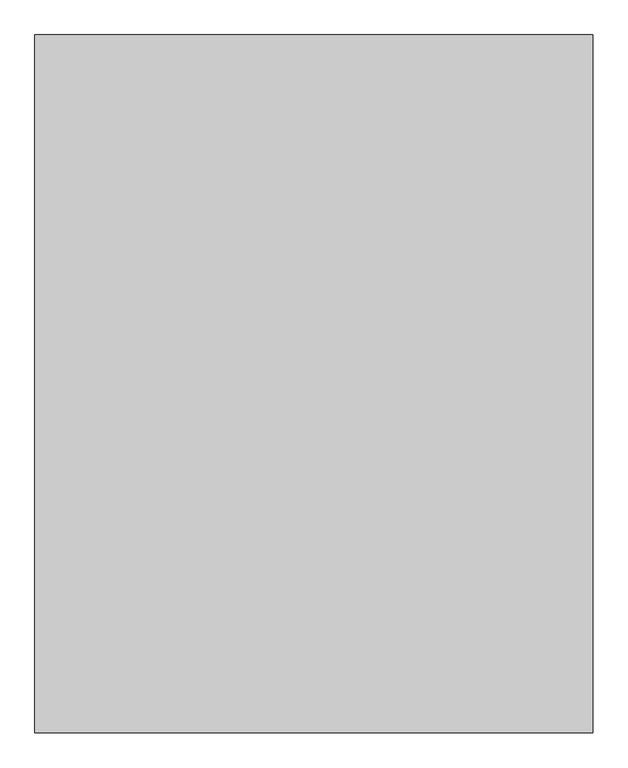
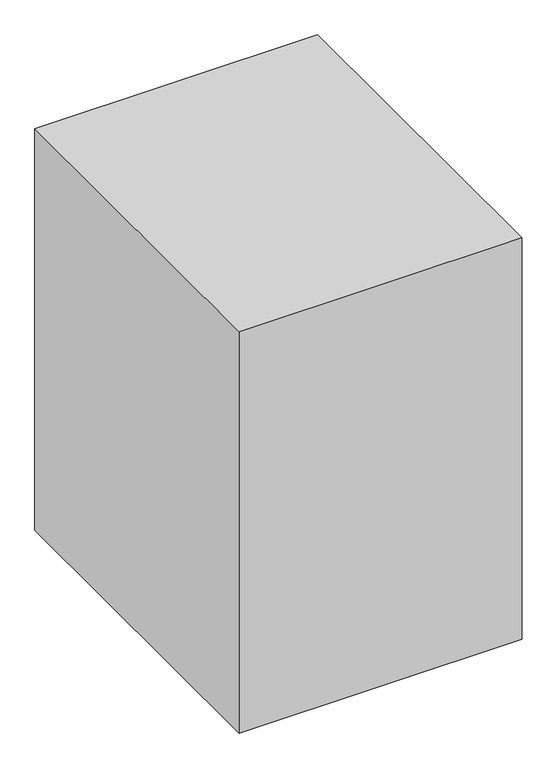
"""IFC4 building model written with IfcOpenShell, lengths in millimetres: proxy geometry, Space Planning Box_hec : Space Planning Box_hec."""

import ifcopenshell
import ifcopenshell.guid

model = None  # the IFC model being written
_history = None  # IfcOwnerHistory: only IFC2X3 demands one
_inside = {}  # id of a spatial element -> (the spatial element, [elements in it])
_under = {}  # id of a project, library or spatial element -> (it, [spatial elements below it])
_declared = {}  # id of a project -> (the project, [libraries it declares])
_typed = {}  # id of a type object -> (the type object, [elements of that type])
_made_of = {}  # id of a material, layer set ... -> (it, [elements and type objects made of it])


def new_model(schema):
    """Start an empty IFC model of exactly this schema.

    Asked for "IFC4X3", IfcOpenShell would pick the latest addendum, in which some entities
    have other attributes; the version numbers below select the first issue.
    IFC2X3 requires an IfcOwnerHistory on every rooted entity: one is made here for all.
    """
    global model, _history
    if schema == "IFC4X3":
        model = ifcopenshell.file(schema_version=(4, 3, 0, 0))
    else:
        model = ifcopenshell.file(schema=schema)
    _inside.clear()
    _under.clear()
    _declared.clear()
    _typed.clear()
    _made_of.clear()
    _history = None
    if model.schema == "IFC2X3":
        org = make("IfcOrganization", Name="unknown")
        user = make(
            "IfcPersonAndOrganization",
            ThePerson=make("IfcPerson", FamilyName="unknown"),
            TheOrganization=org,
        )
        app = make(
            "IfcApplication",
            ApplicationDeveloper=org,
            Version="unknown",
            ApplicationFullName="unknown",
            ApplicationIdentifier="unknown",
        )
        _history = make(
            "IfcOwnerHistory",
            OwningUser=user,
            OwningApplication=app,
            ChangeAction="ADDED",
            CreationDate=0,
        )
    return model


def make(cls, **values):
    """One entity of the class cls with the attributes given. An attribute that is None is left unset."""
    return model.create_entity(
        cls, **{name: value for name, value in values.items() if value is not None}
    )


def rooted(cls, **values):
    """An entity with a GlobalId (a new one), such as an element, a storey or a relation."""
    return make(cls, GlobalId=ifcopenshell.guid.new(), OwnerHistory=_history, **values)


def si_unit(unit_type, name, prefix=None):
    """IfcSIUnit, for example si_unit("LENGTHUNIT", "METRE", prefix="MILLI")."""
    return make("IfcSIUnit", UnitType=unit_type, Prefix=prefix, Name=name)


def assignment(units):
    """IfcUnitAssignment: the units of a project."""
    return None if units is None else make("IfcUnitAssignment", Units=units)


def point(xyz):
    """IfcCartesianPoint."""
    return None if xyz is None else make("IfcCartesianPoint", Coordinates=xyz)


def direction(xyz):
    """IfcDirection."""
    return None if xyz is None else make("IfcDirection", DirectionRatios=xyz)


def frame(location, z_axis=None, x_axis=None):
    """IfcAxis2Placement3D, a coordinate frame: its origin and axes. An axis left out is left unset."""
    return make(
        "IfcAxis2Placement3D",
        Location=point(location),
        Axis=direction(z_axis),
        RefDirection=direction(x_axis),
    )


def origin():
    """The frame at (0, 0, 0) with its axes left unset."""
    return frame((0.0, 0.0, 0.0))


def origin_with_axes():
    """The frame at (0, 0, 0) with the z axis (0, 0, 1) and the x axis (1, 0, 0) written out."""
    return frame((0.0, 0.0, 0.0), z_axis=(0.0, 0.0, 1.0), x_axis=(1.0, 0.0, 0.0))


def place(relative_to, where):
    """IfcLocalPlacement: puts the frame where relative to a parent placement (None: the world)."""
    return make(
        "IfcLocalPlacement", PlacementRelTo=relative_to, RelativePlacement=where
    )


def context(
    kind, dimensions, precision=None, world=None, true_north=None, identifier=None
):
    """IfcGeometricRepresentationContext, for example the 3D "Model" context."""
    return make(
        "IfcGeometricRepresentationContext",
        ContextIdentifier=identifier,
        ContextType=kind,
        CoordinateSpaceDimension=dimensions,
        Precision=precision,
        WorldCoordinateSystem=world,
        TrueNorth=true_north,
    )


def project(units=None, contexts=None):
    """IfcProject with its units and contexts."""
    return rooted(
        "IfcProject",
        Name="project",
        RepresentationContexts=contexts,
        UnitsInContext=assignment(units),
    )


def spatial(cls, under=None, at=None, **own):
    """A site, building, storey or space (cls), placed at a placement, below another one or the project."""
    s = rooted(cls, ObjectPlacement=at, **own)
    if under is not None:
        _under.setdefault(under.id(), (under, []))[1].append(s)
    return s


def polyline(points):
    """IfcPolyline through the points."""
    return make("IfcPolyline", Points=[point(p) for p in points])


def outline(outer, holes=None, kind="AREA"):
    """IfcArbitraryClosedProfileDef: a profile drawn as a closed curve; with holes, ...WithVoids."""
    if holes is None:
        return make("IfcArbitraryClosedProfileDef", ProfileType=kind, OuterCurve=outer)
    return make(
        "IfcArbitraryProfileDefWithVoids",
        ProfileType=kind,
        OuterCurve=outer,
        InnerCurves=holes,
    )


def extrude(swept, where, along, depth):
    """IfcExtrudedAreaSolid: the profile swept, set in the frame where, extruded along a direction by depth."""
    return make(
        "IfcExtrudedAreaSolid",
        SweptArea=swept,
        Position=where,
        ExtrudedDirection=direction(along),
        Depth=depth,
    )


def shape(context_of_items, identifier, shape_type, items):
    """IfcShapeRepresentation: the items that make up one representation, for example the "Body"."""
    return make(
        "IfcShapeRepresentation",
        ContextOfItems=context_of_items,
        RepresentationIdentifier=identifier,
        RepresentationType=shape_type,
        Items=items,
    )


def source(mapping_origin, context_of_items, identifier, shape_type, items):
    """IfcRepresentationMap: a shape defined once, which mapped items show again and again."""
    return make(
        "IfcRepresentationMap",
        MappingOrigin=mapping_origin,
        MappedRepresentation=shape(context_of_items, identifier, shape_type, items),
    )


def transform(
    local_origin,
    x_axis=None,
    y_axis=None,
    z_axis=None,
    scale=None,
    scale2=None,
    scale3=None,
    uniform=True,
):
    """IfcCartesianTransformationOperator3D, or its non-uniform kind. x_axis, y_axis, z_axis: its Axis1, 2, 3."""
    if uniform:
        return make(
            "IfcCartesianTransformationOperator3D",
            Axis1=direction(x_axis),
            Axis2=direction(y_axis),
            LocalOrigin=point(local_origin),
            Scale=scale,
            Axis3=direction(z_axis),
        )
    return make(
        "IfcCartesianTransformationOperator3DnonUniform",
        Axis1=direction(x_axis),
        Axis2=direction(y_axis),
        LocalOrigin=point(local_origin),
        Scale=scale,
        Axis3=direction(z_axis),
        Scale2=scale2,
        Scale3=scale3,
    )


def mapped(mapping_source, mapping_target):
    """IfcMappedItem: shows the shape of a source again, moved by a transform."""
    return make(
        "IfcMappedItem", MappingSource=mapping_source, MappingTarget=mapping_target
    )


def made_of(thing, what):
    """Note that an element or type object is made of a material, layer set ...; save() writes the relation."""
    if what is not None:
        _made_of.setdefault(what.id(), (what, []))[1].append(thing)
    return thing


def element(
    cls,
    number,
    at=None,
    inside=None,
    cuts=None,
    type_object=None,
    material=None,
    context=None,
    identifier="Body",
    shape_type=None,
    held_by="IfcProductDefinitionShape",
    body=None,
    shapes=None,
    **own,
):
    """One element of the class cls, such as IfcWall. Its Tag is "e" and its number.

    at: its placement. inside: the storey or other place that contains it. cuts: it is an
    opening in that element (IfcRelVoidsElement). A single representation is given by context,
    identifier, shape_type and body (its items); several are given by shapes. held_by: the class
    of the entity that holds the representations. save() writes the other relations.
    """
    e = rooted(cls, Tag="e%d" % number, ObjectPlacement=at, **own)
    if body is not None:
        shapes = [shape(context, identifier, shape_type, body)]
    if shapes is not None:
        e.Representation = make(held_by, Representations=shapes)
    if inside is not None:
        _inside.setdefault(inside.id(), (inside, []))[1].append(e)
    if cuts is not None:
        rooted(
            "IfcRelVoidsElement", RelatingBuildingElement=cuts, RelatedOpeningElement=e
        )
    if type_object is not None:
        _typed.setdefault(type_object.id(), (type_object, []))[1].append(e)
    return made_of(e, material)


def aggregate(whole, parts):
    """IfcRelAggregates: a whole, such as a stair, and the parts it consists of."""
    return rooted("IfcRelAggregates", RelatingObject=whole, RelatedObjects=parts)


def save(model, path):
    """Write the relations noted so far, then the file.

    IfcRelAggregates (storeys below a building ...), IfcRelContainedInSpatialStructure (elements
    in a storey), IfcRelDefinesByType, IfcRelAssociatesMaterial and IfcRelDeclares: one each for
    every whole, place, type object, material and project.
    """
    for whole, parts in _under.values():
        aggregate(whole, parts)
    for where, things in _inside.values():
        rooted(
            "IfcRelContainedInSpatialStructure",
            RelatedElements=things,
            RelatingStructure=where,
        )
    for kind, things in _typed.values():
        rooted("IfcRelDefinesByType", RelatedObjects=things, RelatingType=kind)
    for what, things in _made_of.values():
        rooted("IfcRelAssociatesMaterial", RelatedObjects=things, RelatingMaterial=what)
    for by, libraries in _declared.values():
        rooted("IfcRelDeclares", RelatingContext=by, RelatedDefinitions=libraries)
    model.write(path)


def generic_models_5b7b272c(model_context):
    return source(origin(), model_context, "Body", "SweptSolid", [
        extrude(outline(polyline([(2000.0, 2500.0), (2000.0, -2500.0), (-2000.0, -2500.0), (-2000.0, 2500.0), (2000.0, 2500.0)])), origin_with_axes(), (0.0, 0.0, 1.0), 6000.0),
    ])


if __name__ == "__main__":
    model = new_model("IFC4")
    model_context = context("Model", 3, world=origin())
    ifc_project = project(units=[si_unit("LENGTHUNIT", "METRE", prefix="MILLI")], contexts=[model_context])
    site = spatial("IfcSite", under=ifc_project)
    building = spatial("IfcBuilding", under=site)
    placement = place(None, origin())
    generic_models_shape = generic_models_5b7b272c(model_context)
    element("IfcBuildingElementProxy", 1, Name="Space Planning Box_hec : Space Planning Box_hec", ObjectType="Space Planning Box_hec : Space Planning Box_hec", at=placement, inside=building, context=model_context, shape_type="MappedRepresentation", body=[
        mapped(generic_models_shape, transform((0.0, 0.0, 0.0), x_axis=(1.0, 0.0, 0.0), y_axis=(0.0, 1.0, 0.0), z_axis=(0.0, 0.0, 1.0))),
    ])
    save(model, "model.ifc")

# Revit data of these elements
# Type "Space Planning Box_hec : Space Planning Box_hec"
#   Type Comments = "..."
#   Room Name [instance default] = "?"
#   Interior Finish [instance default] = ""
#   Exterior Finish [instance default] = ""
#   Department [instance default] = ""
#   Assembly Code = "..."
#   Width [instance default] = 1524 mm
#   Program Area [instance default] = 0 m²
#   Length [instance default] = 1524 mm
#   Height [instance default] = 1524 mm
#   Area [instance default] = 2.32258 m²
#   Fill Color [instance default] = Cyan
#   Default Elevation = 0
# Element 1 (IfcBuildingElementProxy, "Space Planning Box_hec : Space Planning Box_hec")
#   Room Name = "Toilet (M)"
#   Interior Finish = "IF5"
#   Exterior Finish = "EF1"
#   Department = "AR"
#   Width = 4000 mm
#   Program Area = 72 m²
#   Length = 5000 mm
#   Height = 6000 mm
#   Area = 20 m²
#   Fill Color = Lavender
#   Materials on its faces: "Lavender"
# Materials
#   "Cyan": class "Generic", colour RGB 0 255 255, transparency 0.2, Cost = 0
#   "Lavender": class "Generic", colour RGB 186 85 211, transparency 0.2, Cost = 0
